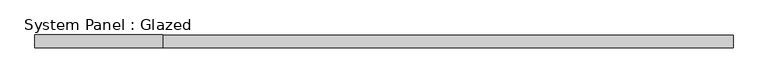
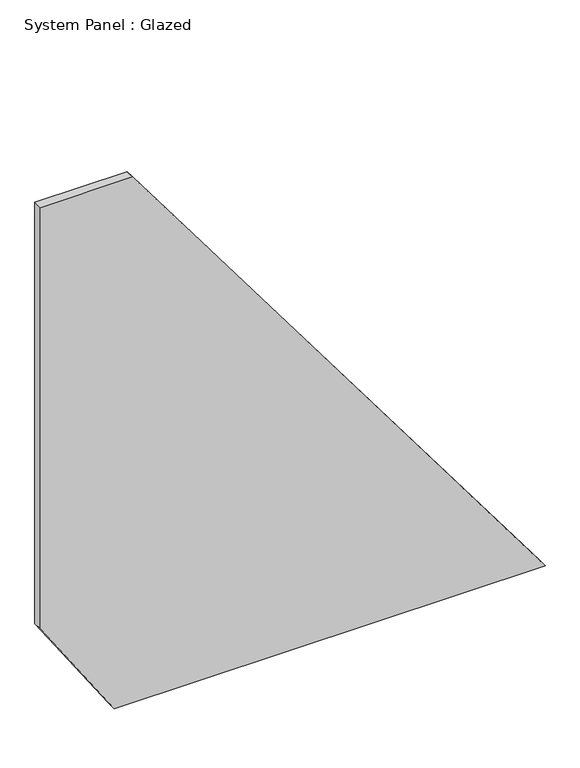
"""IFC4 building model written with IfcOpenShell, lengths in millimetres: plate geometry, System Panel : Glazed."""

from ifc_helpers import new_model, si_unit, frame, origin, place, context, project, spatial, polyline, outline, extrude, source, transform, mapped, element, save


def system_panel_glazed_39dccf24(model_context):
    return source(origin(), model_context, "Body", "SweptSolid", [
        extrude(outline(polyline([(0.0, -482.4313068), (0.0, 682.0985757), (1500.0, -432.7547723), (1500.0, -682.0985757), (297.45995, -682.0985757), (0.0, -482.4313068)])), frame((0.0, 24.5, 0.0), z_axis=(0.0, 1.0, 0.0), x_axis=(0.0, 0.0, 1.0)), (0.0, 0.0, 1.0), 25.0),
    ])


if __name__ == "__main__":
    model = new_model("IFC4")
    model_context = context("Model", 3, world=origin())
    ifc_project = project(units=[si_unit("LENGTHUNIT", "METRE", prefix="MILLI")], contexts=[model_context])
    site = spatial("IfcSite", under=ifc_project)
    building = spatial("IfcBuilding", under=site)
    placement = place(None, origin())
    system_panel_glazed_shape = system_panel_glazed_39dccf24(model_context)
    element("IfcPlate", 1, ObjectType="System Panel : Glazed", at=placement, inside=building, context=model_context, shape_type="MappedRepresentation", body=[
        mapped(system_panel_glazed_shape, transform((0.0, 0.0, 0.0), x_axis=(1.0, 0.0, 0.0), y_axis=(0.0, 1.0, 0.0), z_axis=(0.0, 0.0, 1.0))),
    ])
    save(model, "model.ifc")

# Revit data of these elements
# Type "System Panel : Glazed"
#   Construction Type Id = "GSP4R"
#   Analytic Construction = "1/8 in Pilkington single glazing"
#   Visual Light Transmittance = 0.9
#   Solar Heat Gain Coefficient = 0.86
#   Heat Transfer Coefficient (U) = 6.7069 W/(m²·K)
#   Define Thermal Properties by = 1
# Element 1 (IfcPlate, "System Panel : Glazed")
#   Materials on its faces: "Glass"
# Materials
#   "Glass": class "Glass", colour RGB 0 128 192, transparency 0.9, Description = "Soda Lime Glass", Cost = 0
